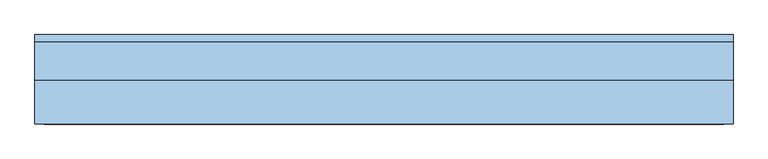
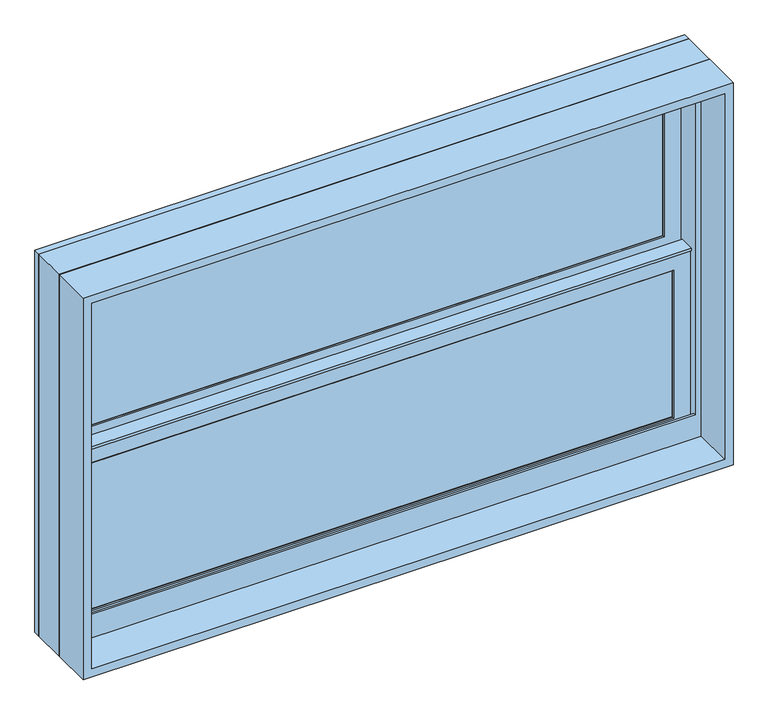
"""IFC4 building model written with IfcOpenShell, lengths in millimetres: window geometry, Window-Double_Hung-Marvin-Essential : ESDH4026."""

from ifc_helpers import new_model, si_unit, frame, origin, place, context, project, spatial, polyline, outline, extrude, faceted_brep, source, transform, mapped, element, save


def window_e550996a(model_context):
    return source(origin(), model_context, "Body", "SolidModel", [
        extrude(outline(polyline([(191.5583333, 20.6375), (191.5583333, 15.875), (172.5083333, 15.875), (172.5083333, 20.6375), (191.5583333, 20.6375)])), frame((0.0, 0.0, 1746.25), z_axis=(0.0, 0.0, 1.0), x_axis=(1.0, 0.0, 0.0)), (0.0, 0.0, 1.0), 298.45),
        extrude(outline(polyline([(-172.5083333, 20.6375), (-172.5083333, 15.875), (-191.5583333, 15.875), (-191.5583333, 20.6375), (-172.5083333, 20.6375)])), frame((0.0, 0.0, 1746.25), z_axis=(0.0, 0.0, 1.0), x_axis=(1.0, 0.0, 0.0)), (0.0, 0.0, 1.0), 298.45),
        extrude(outline(polyline([(546.1, 20.6375), (546.1, 15.875), (-546.1, 15.875), (-546.1, 20.6375), (546.1, 20.6375)])), frame((0.0, 0.0, 1885.95), z_axis=(0.0, 0.0, 1.0), x_axis=(1.0, 0.0, 0.0)), (0.0, 0.0, 1.0), 19.05),
        extrude(outline(polyline([(-191.5583333, 46.83125), (-191.5583333, 51.59375), (-172.5083333, 51.59375), (-172.5083333, 46.83125), (-191.5583333, 46.83125)])), frame((0.0, 0.0, 2082.8), z_axis=(0.0, 0.0, 1.0), x_axis=(1.0, 0.0, 0.0)), (0.0, 0.0, 1.0), 298.45),
        extrude(outline(polyline([(172.5083333, 46.83125), (172.5083333, 51.59375), (191.5583333, 51.59375), (191.5583333, 46.83125), (172.5083333, 46.83125)])), frame((0.0, 0.0, 2082.8), z_axis=(0.0, 0.0, 1.0), x_axis=(1.0, 0.0, 0.0)), (0.0, 0.0, 1.0), 298.45),
        extrude(outline(polyline([(-546.1, 46.83125), (-546.1, 51.59375), (546.1, 51.59375), (546.1, 46.83125), (-546.1, 46.83125)])), frame((0.0, 0.0, 2222.5), z_axis=(0.0, 0.0, 1.0), x_axis=(1.0, 0.0, 0.0)), (0.0, 0.0, 1.0), 19.05),
        extrude(outline(polyline([(191.5583333, 20.6375), (172.5083333, 20.6375), (172.5083333, 25.4), (191.5583333, 25.4), (191.5583333, 20.6375)])), frame((0.0, 0.0, 1746.25), z_axis=(0.0, 0.0, 1.0), x_axis=(1.0, 0.0, 0.0)), (0.0, 0.0, 1.0), 298.45),
        extrude(outline(polyline([(-172.5083333, 20.6375), (-191.5583333, 20.6375), (-191.5583333, 25.4), (-172.5083333, 25.4), (-172.5083333, 20.6375)])), frame((0.0, 0.0, 1746.25), z_axis=(0.0, 0.0, 1.0), x_axis=(1.0, 0.0, 0.0)), (0.0, 0.0, 1.0), 298.45),
        extrude(outline(polyline([(546.1, 20.6375), (-546.1, 20.6375), (-546.1, 25.4), (546.1, 25.4), (546.1, 20.6375)])), frame((0.0, 0.0, 1885.95), z_axis=(0.0, 0.0, 1.0), x_axis=(1.0, 0.0, 0.0)), (0.0, 0.0, 1.0), 19.05),
        extrude(outline(polyline([(-191.5583333, 56.35625), (-172.5083333, 56.35625), (-172.5083333, 51.59375), (-191.5583333, 51.59375), (-191.5583333, 56.35625)])), frame((0.0, 0.0, 2082.8), z_axis=(0.0, 0.0, 1.0), x_axis=(1.0, 0.0, 0.0)), (0.0, 0.0, 1.0), 298.45),
        extrude(outline(polyline([(172.5083333, 56.35625), (191.5583333, 56.35625), (191.5583333, 51.59375), (172.5083333, 51.59375), (172.5083333, 56.35625)])), frame((0.0, 0.0, 2082.8), z_axis=(0.0, 0.0, 1.0), x_axis=(1.0, 0.0, 0.0)), (0.0, 0.0, 1.0), 298.45),
        extrude(outline(polyline([(-546.1, 56.35625), (546.1, 56.35625), (546.1, 51.59375), (-546.1, 51.59375), (-546.1, 56.35625)])), frame((0.0, 0.0, 2222.5), z_axis=(0.0, 0.0, 1.0), x_axis=(1.0, 0.0, 0.0)), (0.0, 0.0, 1.0), 19.05),
        faceted_brep([(-573.0875, 5.6780605, 2074.7351748), (-573.0875, 5.6780605, 2070.1), (573.0875, 5.6780605, 2070.1), (573.0875, 5.6780605, 2074.7351748), (-573.0875, 34.8118605, 2074.7351748), (573.0875, 34.8118605, 2074.7351748), (573.0875, 34.8118605, 2070.1), (-573.0875, 34.8118605, 2070.1), (-573.0875, 30.1625, 2070.1), (-573.0875, 30.1625, 1719.2625), (-573.0875, 8.9241104, 1719.2625), (-573.0875, 8.9241104, 2070.1), (573.0875, 8.9241104, 2070.1), (573.0875, 30.1625, 2070.1), (573.0875, 8.9241104, 1719.2625), (573.0875, 30.1625, 1719.2625), (-557.2034752, 11.90625, 2055.8034752), (-557.2034752, 30.1625, 2055.8034752), (557.2034752, 30.1625, 2055.8034752), (557.2034752, 11.90625, 2055.8034752), (-540.54375, 10.4662439, 2039.14375), (-540.54375, 11.90625, 2039.14375), (540.54375, 11.90625, 2039.14375), (540.54375, 10.4662439, 2039.14375), (542.0858834, 8.9241104, 2040.6858834), (-542.0858834, 8.9241104, 2040.6858834), (557.2034752, 30.1625, 1735.1465248), (557.2034752, 11.90625, 1735.1465248), (540.54375, 11.90625, 1751.80625), (540.54375, 10.4662439, 1751.80625), (542.0858834, 8.9241104, 1750.2641166), (-557.2034752, 30.1625, 1735.1465248), (-557.2034752, 11.90625, 1735.1465248), (-540.54375, 11.90625, 1751.80625), (-540.54375, 10.4662439, 1751.80625), (-542.0858834, 8.9241104, 1750.2641166)], [[[0, 1, 2, 3]], [[4, 5, 6, 7]], [[1, 0, 4, 7, 8, 9, 10, 11]], [[2, 1, 11, 12]], [[7, 6, 13, 8]], [[3, 2, 12, 14, 15, 13, 6, 5]], [[0, 3, 5, 4]], [[16, 17, 18, 19]], [[20, 21, 22, 23]], [[20, 23, 24, 25]], [[19, 18, 26, 27]], [[23, 22, 28, 29]], [[24, 23, 29, 30]], [[27, 26, 31, 32]], [[29, 28, 33, 34]], [[30, 29, 34, 35]], [[15, 14, 10, 9]], [[15, 9, 8, 13], [18, 17, 31, 26]], [[17, 16, 32, 31]], [[16, 19, 27, 32], [22, 21, 33, 28]], [[21, 20, 34, 33]], [[20, 25, 35, 34]], [[10, 14, 12, 11], [25, 24, 30, 35]]]),
        extrude(outline(polyline([(38.5955581, 2055.8125), (33.5778968, 2055.8125), (33.5778968, 2057.4), (39.9405976, 2057.4), (39.9405976, 2055.8125), (61.515625, 2055.8125), (47.6307501, 2052.4975159), (38.5955581, 2052.4975159), (38.5955581, 2055.8125)])), frame((-573.0875, 0.0, 0.0), z_axis=(1.0, 0.0, 0.0), x_axis=(0.0, 1.0, 0.0)), (0.0, 0.0, 1.0), 1146.175),
        faceted_brep([(603.25, 0.0, 1689.1), (603.25, 0.0, 2438.4), (-603.25, 0.0, 2438.4), (-603.25, 0.0, 1689.1), (577.05625, 0.0, 1750.21875), (-577.05625, 0.0, 1750.21875), (-577.05625, 0.0, 2412.20625), (577.05625, 0.0, 2412.20625), (577.05625, 3.96875, 1689.1), (-577.05625, 3.96875, 1689.1), (-577.05625, 3.96875, 1750.21875), (577.05625, 3.96875, 1750.21875), (-603.25, 65.6828125, 1689.1), (-577.05625, 65.6828125, 1689.1), (577.05625, 65.6828125, 1689.1), (603.25, 65.6828125, 1689.1), (-603.25, 65.6828125, 2438.4), (603.25, 65.6828125, 2438.4), (577.05625, 65.6828125, 2412.20625), (-577.05625, 65.6828125, 2412.20625)], [[[0, 1, 2, 3], [4, 5, 6, 7]], [[8, 9, 10, 11]], [[5, 4, 11, 10]], [[0, 3, 12, 13, 9, 8, 14, 15]], [[13, 12, 16, 17, 15, 14, 18, 19]], [[13, 19, 6, 5, 10, 9]], [[7, 6, 19, 18]], [[18, 14, 8, 11, 4, 7]], [[1, 0, 15, 17]], [[2, 1, 17, 16]], [[3, 2, 16, 12]]]),
        faceted_brep([(577.05625, 30.1625, 2063.75), (575.46875, 30.1625, 2063.75), (575.46875, 30.1625, 1713.4544613), (577.05625, 30.1625, 1713.4544613), (-575.46875, 30.1625, 2063.75), (-577.05625, 30.1625, 2063.75), (-577.05625, 30.1625, 1713.4544613), (-575.46875, 30.1625, 1713.4544613), (575.46875, 63.5, 2063.75), (577.05625, 63.5, 2063.75), (577.05625, 63.5, 1706.9743077), (575.46875, 63.5, 1706.9743077), (-577.05625, 63.5, 2063.75), (-575.46875, 63.5, 2063.75), (-575.46875, 63.5, 1706.9743077), (-577.05625, 63.5, 1706.9743077), (588.3108932, 3.96875, 1718.5460105), (588.3108932, 3.96875, 1689.1), (588.3108932, 65.6828125, 1689.1), (588.3108932, 65.6828125, 1706.550012), (-588.3108932, 3.96875, 1689.1), (-588.3108932, 3.96875, 1718.5460105), (-588.3108932, 65.6828125, 1706.550012), (-588.3108932, 65.6828125, 1689.1), (588.3108932, 78.58125, 1704.0428097), (-588.3108932, 78.58125, 1704.0428097), (-586.2971252, 68.2348864, 1706.0539391), (-568.33135, 68.2348864, 1706.0539391), (-568.33135, 65.6828125, 1706.550012), (568.33135, 65.6828125, 1706.550012), (568.33135, 68.2348864, 1706.0539391), (586.2971252, 68.2348864, 1706.0539391), (-603.25, 65.6828125, 1689.1), (-603.25, 78.5948249, 1689.1), (603.25, 78.5948249, 1689.1), (603.25, 65.6828125, 1689.1), (-603.25, 78.58125, 2438.4), (603.25, 78.58125, 2438.4), (588.3108932, 78.58125, 2423.4608932), (-588.3108932, 78.58125, 2423.4608932), (-603.25, 65.6828125, 2438.4), (-586.2971252, 68.2348864, 2421.4471252), (586.2971252, 68.2348864, 2421.4471252), (568.33135, 68.2348864, 2403.48135), (-568.33135, 68.2348864, 2403.48135), (-568.33135, 65.6828125, 2403.48135), (568.33135, 65.6828125, 2403.48135), (603.25, 65.6828125, 2438.4)], [[[0, 1, 2, 3]], [[4, 5, 6, 7]], [[8, 9, 10, 11]], [[12, 13, 14, 15]], [[1, 8, 11, 2]], [[9, 0, 3, 10]], [[1, 0, 9, 8]], [[5, 4, 13, 12]], [[5, 12, 15, 6]], [[13, 4, 7, 14]], [[16, 17, 18, 19]], [[20, 21, 22, 23]], [[24, 25, 26, 27, 28, 22, 21, 16, 19, 29, 30, 31], [3, 2, 11, 10], [7, 6, 15, 14]], [[17, 16, 21, 20]], [[17, 20, 23, 32, 33, 34, 35, 18]], [[34, 33, 36, 37], [25, 24, 38, 39]], [[33, 32, 40, 36]], [[39, 41, 26, 25]], [[41, 42, 31, 30, 43, 44, 27, 26]], [[44, 45, 28, 27]], [[40, 32, 23, 22, 28, 45, 46, 29, 19, 18, 35, 47]], [[36, 40, 47, 37]], [[39, 38, 42, 41]], [[44, 43, 46, 45]], [[34, 37, 47, 35]], [[42, 38, 24, 31]], [[46, 43, 30, 29]]]),
        extrude(outline(polyline([(553.24375, 11.90625), (-553.24375, 11.90625), (-553.24375, 15.08125), (553.24375, 15.08125), (553.24375, 11.90625)])), frame((0.0, 0.0, 1739.10625), z_axis=(0.0, 0.0, 1.0), x_axis=(1.0, 0.0, 0.0)), (0.0, 0.0, 1.0), 312.7375),
        extrude(outline(polyline([(553.24375, 42.8625), (-553.24375, 42.8625), (-553.24375, 46.0375), (553.24375, 46.0375), (553.24375, 42.8625)])), frame((0.0, 0.0, 2075.65625), z_axis=(0.0, 0.0, 1.0), x_axis=(1.0, 0.0, 0.0)), (0.0, 0.0, 1.0), 312.7375),
        faceted_brep([(-540.54375, 31.194477, 2039.14375), (-542.0858834, 32.7366104, 2040.6858834), (542.0858834, 32.7366104, 2040.6858834), (540.54375, 31.194477, 2039.14375), (-540.54375, 30.1625, 2039.14375), (540.54375, 30.1625, 2039.14375), (-573.0875, 32.7366104, 2071.6875), (-573.0875, 30.1625, 2071.6875), (573.0875, 30.1625, 2071.6875), (573.0875, 32.7366104, 2071.6875), (542.0858834, 32.7366104, 1750.2641166), (540.54375, 31.194477, 1751.80625), (540.54375, 30.1625, 1751.80625), (573.0875, 30.1625, 1719.2625), (573.0875, 32.7366104, 1719.2625), (-542.0858834, 32.7366104, 1750.2641166), (-540.54375, 31.194477, 1751.80625), (-540.54375, 30.1625, 1751.80625), (-573.0875, 30.1625, 1719.2625), (-573.0875, 32.7366104, 1719.2625)], [[[0, 1, 2, 3]], [[4, 0, 3, 5]], [[6, 7, 8, 9]], [[3, 2, 10, 11]], [[5, 3, 11, 12]], [[9, 8, 13, 14]], [[11, 10, 15, 16]], [[12, 11, 16, 17]], [[14, 13, 18, 19]], [[9, 14, 19, 6], [1, 15, 10, 2]], [[16, 15, 1, 0]], [[17, 16, 0, 4]], [[7, 18, 13, 8], [5, 12, 17, 4]], [[19, 18, 7, 6]]]),
        faceted_brep([(-557.2034752, 42.8625, 2392.3534752), (-557.2034752, 61.11875, 2392.3534752), (557.2034752, 61.11875, 2392.3534752), (557.2034752, 42.8625, 2392.3534752), (-540.54375, 41.4224939, 2375.69375), (-540.54375, 42.8625, 2375.69375), (540.54375, 42.8625, 2375.69375), (540.54375, 41.4224939, 2375.69375), (-542.0858834, 39.8803604, 2377.2358834), (542.0858834, 39.8803604, 2377.2358834), (-573.0875, 61.11875, 2408.2375), (-573.0875, 39.8803604, 2408.2375), (573.0875, 39.8803604, 2408.2375), (573.0875, 61.11875, 2408.2375), (557.2034752, 61.11875, 2071.6965248), (557.2034752, 42.8625, 2071.6965248), (540.54375, 42.8625, 2088.35625), (540.54375, 41.4224939, 2088.35625), (542.0858834, 39.8803604, 2086.8141166), (573.0875, 39.8803604, 2055.8125), (573.0875, 61.11875, 2055.8125), (-557.2034752, 61.11875, 2071.6965248), (-557.2034752, 42.8625, 2071.6965248), (-540.54375, 42.8625, 2088.35625), (-540.54375, 41.4224939, 2088.35625), (-542.0858834, 39.8803604, 2086.8141166), (-573.0875, 39.8803604, 2055.8125), (-573.0875, 61.11875, 2055.8125)], [[[0, 1, 2, 3]], [[4, 5, 6, 7]], [[8, 4, 7, 9]], [[10, 11, 12, 13]], [[3, 2, 14, 15]], [[7, 6, 16, 17]], [[9, 7, 17, 18]], [[13, 12, 19, 20]], [[15, 14, 21, 22]], [[17, 16, 23, 24]], [[18, 17, 24, 25]], [[20, 19, 26, 27]], [[13, 20, 27, 10], [1, 21, 14, 2]], [[22, 21, 1, 0]], [[3, 15, 22, 0], [5, 23, 16, 6]], [[24, 23, 5, 4]], [[25, 24, 4, 8]], [[11, 26, 19, 12], [9, 18, 25, 8]], [[27, 26, 11, 10]]]),
        faceted_brep([(-573.0875, 61.11875, 2055.8125), (-573.0875, 63.6928604, 2055.8125), (573.0875, 63.6928604, 2055.8125), (573.0875, 61.11875, 2055.8125), (-540.54375, 62.150727, 2088.35625), (-540.54375, 61.11875, 2088.35625), (540.54375, 61.11875, 2088.35625), (540.54375, 62.150727, 2088.35625), (-542.0858834, 63.6928604, 2086.8141166), (542.0858834, 63.6928604, 2086.8141166), (573.0875, 63.6928604, 2408.2375), (573.0875, 61.11875, 2408.2375), (540.54375, 61.11875, 2375.69375), (540.54375, 62.150727, 2375.69375), (542.0858834, 63.6928604, 2377.2358834), (-573.0875, 63.6928604, 2408.2375), (-573.0875, 61.11875, 2408.2375), (-540.54375, 61.11875, 2375.69375), (-540.54375, 62.150727, 2375.69375), (-542.0858834, 63.6928604, 2377.2358834)], [[[0, 1, 2, 3]], [[4, 5, 6, 7]], [[8, 4, 7, 9]], [[3, 2, 10, 11]], [[7, 6, 12, 13]], [[9, 7, 13, 14]], [[11, 10, 15, 16]], [[13, 12, 17, 18]], [[14, 13, 18, 19]], [[16, 15, 1, 0]], [[3, 11, 16, 0], [5, 17, 12, 6]], [[18, 17, 5, 4]], [[19, 18, 4, 8]], [[1, 15, 10, 2], [9, 14, 19, 8]]]),
        extrude(outline(polyline([(553.24375, 26.19375), (-553.24375, 26.19375), (-553.24375, 30.1625), (553.24375, 30.1625), (553.24375, 26.19375)])), frame((0.0, 0.0, 1739.10625), z_axis=(0.0, 0.0, 1.0), x_axis=(1.0, 0.0, 0.0)), (0.0, 0.0, 1.0), 312.7375),
        extrude(outline(polyline([(553.24375, 57.15), (-553.24375, 57.15), (-553.24375, 61.11875), (553.24375, 61.11875), (553.24375, 57.15)])), frame((0.0, 0.0, 2075.65625), z_axis=(0.0, 0.0, 1.0), x_axis=(1.0, 0.0, 0.0)), (0.0, 0.0, 1.0), 312.7375),
        extrude(outline(polyline([(2438.4, 603.25), (2438.4, -603.25), (1689.1, -603.25), (1689.1, 603.25), (2438.4, 603.25)]), holes=[polyline([(2422.525, 587.375), (1704.975, 587.375), (1704.975, -587.375), (2422.525, -587.375), (2422.525, 587.375)])]), frame((0.0, -76.2, 0.0), z_axis=(0.0, 1.0, 0.0), x_axis=(0.0, 0.0, 1.0)), (0.0, 0.0, 1.0), 75.40625),
    ])


if __name__ == "__main__":
    model = new_model("IFC4")
    model_context = context("Model", 3, world=origin())
    ifc_project = project(units=[si_unit("LENGTHUNIT", "METRE", prefix="MILLI")], contexts=[model_context])
    site = spatial("IfcSite", under=ifc_project)
    building = spatial("IfcBuilding", under=site)
    placement = place(None, origin())
    window_shape = window_e550996a(model_context)
    element("IfcWindow", 1, ObjectType="Window-Double_Hung-Marvin-Essential : ESDH4026", at=placement, inside=building, context=model_context, shape_type="MappedRepresentation", body=[
        mapped(window_shape, transform((0.0, 0.0, 0.0), x_axis=(1.0, 0.0, 0.0), y_axis=(0.0, 1.0, 0.0), z_axis=(0.0, 0.0, 1.0))),
    ])
    save(model, "model.ifc")

# Revit data of these elements
# Type "Window-Double_Hung-Marvin-Essential : ESDH4026"
#   Type Mark = "32"
#   Window Type = "Essential Double Hung"
#   Product data url = "https://bimobject.com/marvin-windows-and-doors/product/marvin-dhwau"
#   Product Guid = "c4a96547-874c-4385-91dc-a058adc19d98"
#   Frame = "All Ultrex"
#   Egress Window = "No"
#   URL = "www.marvin.com"
#   Model = "ESDH4026"
#   Manufacturer = "Marvin Windows and Doors"
#   Label Egress = ""
#   Glass Type = "IG Low E II with Argon"
#   Design Pressure = "DP50"
#   Description = "4830 DBHG"
#   Analytic Construction = "<None>"
#   Prairie Corner Width = 0' - 4"
#   Prairie Corner Height = 0' - 4"
#   Egress Width = 3' - 8 9/16"
#   Egress Height = 0' - 10 27/128"
#   Rough Width = 4' - 0"
#   Rough Height = 2' - 6"
#   Nominal Width = 4' - 0"
#   Nominal Height = 2' - 6"
#   Inset to Installation Flange [instance default] = 0' - 1"
#   Height = 2' - 5 1/2"
#   Egress Area = 3.1599 SF
#   Default Head Height = 8' - 0"
#   Width = 3' - 11 1/2"
#   Daylight Area = 6.68734 SF
#   DLO Width = 3' - 6 9/16"
#   DLO Height = 0' - 11 5/16"
#   Muntins Top Sash = yes
#   Lites Wide Top Sash = 3
#   Lites Wide Bottom Sash = 3
#   Lites High Top Sash = 2
#   Lites High Bottom Sash = 2
#   Lite Cut Prairie 9 = no
#   Lite Cut HV Grid = yes
#   Muntins Bottom Sash = yes
#   Label Visibility = no
#   Jamb Extension Visibility = yes
#   Edition number = 1
#   Interior Material = Ultrex-Marvin-Stonewhite
#   Glazing Material = Glass-Marvin-IG Low E II with Argon
#   Cladding Material = Ultrex-Marvin-Pebblegray
#   Wall Closure = (empty or 0)
#   Assembly Code = ""
# Element 1 (IfcWindow, "Window-Double_Hung-Marvin-Essential : ESDH4026")
#   Materials on its faces: "Ultrex-Marvin-Pebblegray", "Ultrex-Marvin-Stonewhite", "Glass-Marvin-IG Low E II with Argon"
# Materials
#   "Ultrex-Marvin-Stonewhite": class "Paint", colour RGB 250 251 245, transparency 0
#   "Glass-Marvin-IG Low E II with Argon": class "Glass", colour RGB 0 128 192, transparency 0.85
#   "Ultrex-Marvin-Pebblegray": class "Paint", colour RGB 189 185 173, transparency 0
